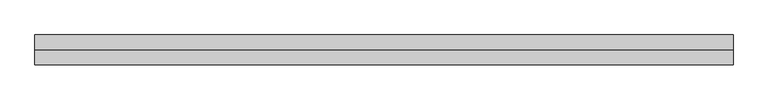
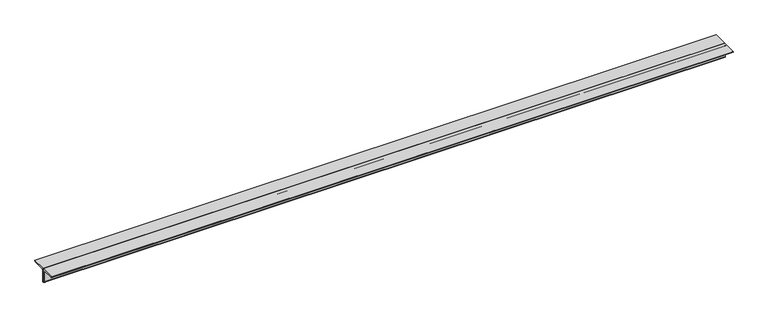
"""IFC4 building model written with IfcOpenShell, lengths in millimetres: beam geometry, 0123_Steel Framing_2Ls-KSD3502 : H_SB_AR_S04_2Ls-130x130x12_VBR2."""

from ifc_helpers import new_model, si_unit, point, frame, frame_2d, origin, place, context, project, spatial, polyline, circle_curve, trimmed, segment, composite_curve, outline, extrude, source, transform, mapped, element, save


def beam_a61622f5(model_context):
    return source(origin(), model_context, "Body", "SweptSolid", [
        extrude(outline(composite_curve([segment(polyline([(0.0, 36.4), (130.0, 36.4)]), True, "CONTINUOUS"), segment(trimmed(circle_curve(frame_2d((118.0, 36.4)), 12.0), [point((130.0, 36.4))], [point((118.0, 24.4))], False, "CARTESIAN"), True, "CONTINUOUS"), segment(polyline([(118.0, 24.4), (24.0, 24.4)]), True, "CONTINUOUS"), segment(trimmed(circle_curve(frame_2d((24.0, 12.4)), 12.0), [point((24.0, 24.4))], [point((12.0, 12.4))], True, "CARTESIAN"), True, "CONTINUOUS"), segment(polyline([(12.0, 12.4), (12.0, -81.6)]), True, "CONTINUOUS"), segment(trimmed(circle_curve(frame_2d((0.0, -81.6)), 12.0), [point((12.0, -81.6))], [point((0.0, -93.6))], False, "CARTESIAN"), True, "CONTINUOUS"), segment(polyline([(0.0, -93.6), (0.0, 36.4)]), True, "CONTINUOUS")], self_intersect=False)), frame((-3093.2366876, 0.0, 0.0), z_axis=(1.0, 0.0, 0.0), x_axis=(0.0, 1.0, 0.0)), (0.0, 0.0, 1.0), 6055.217292),
        extrude(outline(composite_curve([segment(polyline([(0.0, 36.4), (0.0, -93.6)]), True, "CONTINUOUS"), segment(trimmed(circle_curve(frame_2d((0.0, -81.6)), 12.0), [point((0.0, -93.6))], [point((-12.0, -81.6))], False, "CARTESIAN"), True, "CONTINUOUS"), segment(polyline([(-12.0, -81.6), (-12.0, 12.4)]), True, "CONTINUOUS"), segment(trimmed(circle_curve(frame_2d((-24.0, 12.4)), 12.0), [point((-12.0, 12.4))], [point((-24.0, 24.4))], True, "CARTESIAN"), True, "CONTINUOUS"), segment(polyline([(-24.0, 24.4), (-118.0, 24.4)]), True, "CONTINUOUS"), segment(trimmed(circle_curve(frame_2d((-118.0, 36.4)), 12.0), [point((-118.0, 24.4))], [point((-130.0, 36.4))], False, "CARTESIAN"), True, "CONTINUOUS"), segment(polyline([(-130.0, 36.4), (0.0, 36.4)]), True, "CONTINUOUS")], self_intersect=False)), frame((-3093.2366876, 0.0, 0.0), z_axis=(1.0, 0.0, 0.0), x_axis=(0.0, 1.0, 0.0)), (0.0, 0.0, 1.0), 6055.217292),
    ])


if __name__ == "__main__":
    model = new_model("IFC4")
    model_context = context("Model", 3, world=origin())
    ifc_project = project(units=[si_unit("LENGTHUNIT", "METRE", prefix="MILLI")], contexts=[model_context])
    site = spatial("IfcSite", under=ifc_project)
    building = spatial("IfcBuilding", under=site)
    placement = place(None, origin())
    beam_shape = beam_a61622f5(model_context)
    element("IfcBeam", 1, ObjectType="0123_Steel Framing_2Ls-KSD3502 : H_SB_AR_S04_2Ls-130x130x12_VBR2", at=placement, inside=building, context=model_context, shape_type="MappedRepresentation", body=[
        mapped(beam_shape, transform((0.0, 0.0, 0.0), x_axis=(1.0, 0.0, 0.0), y_axis=(0.0, 1.0, 0.0), z_axis=(0.0, 0.0, 1.0))),
    ])
    save(model, "model.ifc")

# Revit data of these elements
# Type "0123_Steel Framing_2Ls-KSD3502 : H_SB_AR_S04_2Ls-130x130x12_VBR2"
#   Type Mark = "VBR2"
#   Assembly Code = "B10"
#   Legs = "SLBB"
#   W = 8.97
#   Perimeter = 1.04 m²/m
#   Nominal Weight = 46.80 kgf/m
#   Length [instance default] = 1000 mm
#   Space = 0 mm
#   b = 130 mm
#   d = 130 mm
#   t = 12 mm
#   y = 36.4 mm
#   A = 0.005952 m²
#   Structural Material [instance default] = Steel ASTM A36
# Element 1 (IfcBeam, "0123_Steel Framing_2Ls-KSD3502 : H_SB_AR_S04_2Ls-130x130x12_VBR2")
#   Materials on its faces: "Steel ASTM A36"
# Materials
#   "Steel ASTM A36": class "Metal", colour RGB 199 199 199, transparency 0, Description = "Structural steel, ASTM A36 Grade B, mill finish", Cost = 0
